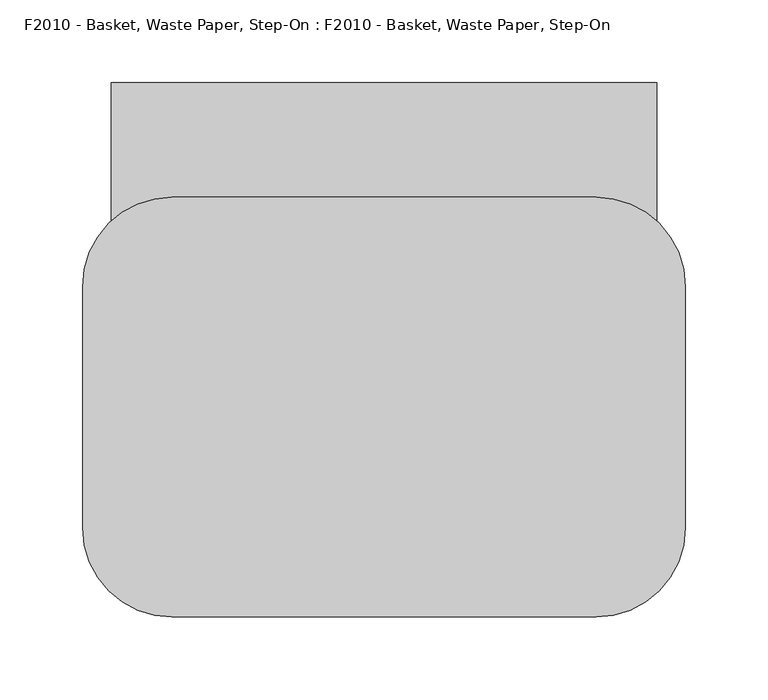
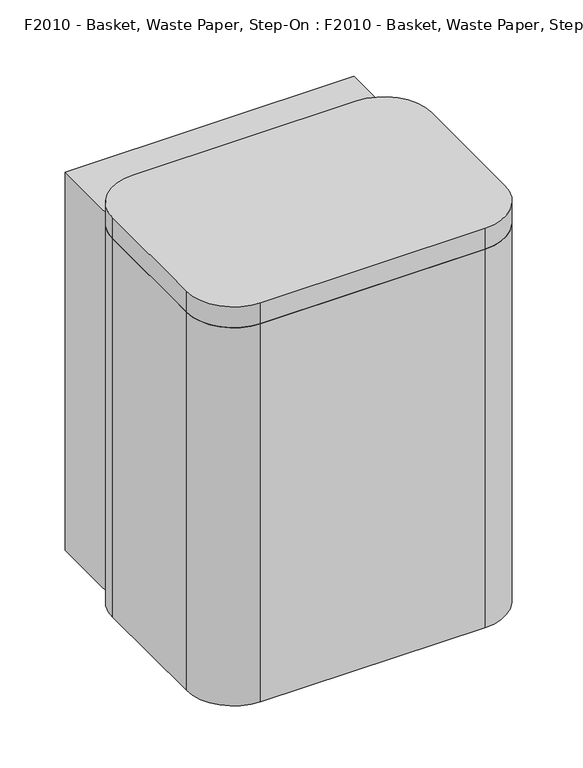
"""IFC4 building model written with IfcOpenShell, lengths in millimetres: proxy geometry, F2010 - Basket, Waste Paper, Step-On : F2010 - Basket, Waste Paper, Step-On."""

import ifcopenshell
import ifcopenshell.guid

model = None  # the IFC model being written
_history = None  # IfcOwnerHistory: only IFC2X3 demands one
_inside = {}  # id of a spatial element -> (the spatial element, [elements in it])
_under = {}  # id of a project, library or spatial element -> (it, [spatial elements below it])
_declared = {}  # id of a project -> (the project, [libraries it declares])
_typed = {}  # id of a type object -> (the type object, [elements of that type])
_made_of = {}  # id of a material, layer set ... -> (it, [elements and type objects made of it])


def new_model(schema):
    """Start an empty IFC model of exactly this schema.

    Asked for "IFC4X3", IfcOpenShell would pick the latest addendum, in which some entities
    have other attributes; the version numbers below select the first issue.
    IFC2X3 requires an IfcOwnerHistory on every rooted entity: one is made here for all.
    """
    global model, _history
    if schema == "IFC4X3":
        model = ifcopenshell.file(schema_version=(4, 3, 0, 0))
    else:
        model = ifcopenshell.file(schema=schema)
    _inside.clear()
    _under.clear()
    _declared.clear()
    _typed.clear()
    _made_of.clear()
    _history = None
    if model.schema == "IFC2X3":
        org = make("IfcOrganization", Name="unknown")
        user = make(
            "IfcPersonAndOrganization",
            ThePerson=make("IfcPerson", FamilyName="unknown"),
            TheOrganization=org,
        )
        app = make(
            "IfcApplication",
            ApplicationDeveloper=org,
            Version="unknown",
            ApplicationFullName="unknown",
            ApplicationIdentifier="unknown",
        )
        _history = make(
            "IfcOwnerHistory",
            OwningUser=user,
            OwningApplication=app,
            ChangeAction="ADDED",
            CreationDate=0,
        )
    return model


def make(cls, **values):
    """One entity of the class cls with the attributes given. An attribute that is None is left unset."""
    return model.create_entity(
        cls, **{name: value for name, value in values.items() if value is not None}
    )


def rooted(cls, **values):
    """An entity with a GlobalId (a new one), such as an element, a storey or a relation."""
    return make(cls, GlobalId=ifcopenshell.guid.new(), OwnerHistory=_history, **values)


def si_unit(unit_type, name, prefix=None):
    """IfcSIUnit, for example si_unit("LENGTHUNIT", "METRE", prefix="MILLI")."""
    return make("IfcSIUnit", UnitType=unit_type, Prefix=prefix, Name=name)


def assignment(units):
    """IfcUnitAssignment: the units of a project."""
    return None if units is None else make("IfcUnitAssignment", Units=units)


def point(xyz):
    """IfcCartesianPoint."""
    return None if xyz is None else make("IfcCartesianPoint", Coordinates=xyz)


def direction(xyz):
    """IfcDirection."""
    return None if xyz is None else make("IfcDirection", DirectionRatios=xyz)


def frame(location, z_axis=None, x_axis=None):
    """IfcAxis2Placement3D, a coordinate frame: its origin and axes. An axis left out is left unset."""
    return make(
        "IfcAxis2Placement3D",
        Location=point(location),
        Axis=direction(z_axis),
        RefDirection=direction(x_axis),
    )


def frame_2d(location, x_axis=None):
    """IfcAxis2Placement2D, a coordinate frame in the plane: its origin and x axis."""
    return make(
        "IfcAxis2Placement2D", Location=point(location), RefDirection=direction(x_axis)
    )


def origin():
    """The frame at (0, 0, 0) with its axes left unset."""
    return frame((0.0, 0.0, 0.0))


def origin_with_axes():
    """The frame at (0, 0, 0) with the z axis (0, 0, 1) and the x axis (1, 0, 0) written out."""
    return frame((0.0, 0.0, 0.0), z_axis=(0.0, 0.0, 1.0), x_axis=(1.0, 0.0, 0.0))


def place(relative_to, where):
    """IfcLocalPlacement: puts the frame where relative to a parent placement (None: the world)."""
    return make(
        "IfcLocalPlacement", PlacementRelTo=relative_to, RelativePlacement=where
    )


def context(
    kind, dimensions, precision=None, world=None, true_north=None, identifier=None
):
    """IfcGeometricRepresentationContext, for example the 3D "Model" context."""
    return make(
        "IfcGeometricRepresentationContext",
        ContextIdentifier=identifier,
        ContextType=kind,
        CoordinateSpaceDimension=dimensions,
        Precision=precision,
        WorldCoordinateSystem=world,
        TrueNorth=true_north,
    )


def project(units=None, contexts=None):
    """IfcProject with its units and contexts."""
    return rooted(
        "IfcProject",
        Name="project",
        RepresentationContexts=contexts,
        UnitsInContext=assignment(units),
    )


def spatial(cls, under=None, at=None, **own):
    """A site, building, storey or space (cls), placed at a placement, below another one or the project."""
    s = rooted(cls, ObjectPlacement=at, **own)
    if under is not None:
        _under.setdefault(under.id(), (under, []))[1].append(s)
    return s


def polyline(points):
    """IfcPolyline through the points."""
    return make("IfcPolyline", Points=[point(p) for p in points])


def circle_curve(where, radius):
    """IfcCircle in the frame where."""
    return make("IfcCircle", Position=where, Radius=radius)


def trimmed(basis, trim1, trim2, sense, master):
    """IfcTrimmedCurve: the piece of a basis curve between two trims."""
    return make(
        "IfcTrimmedCurve",
        BasisCurve=basis,
        Trim1=trim1,
        Trim2=trim2,
        SenseAgreement=sense,
        MasterRepresentation=master,
    )


def segment(curve, same_sense, transition):
    """IfcCompositeCurveSegment."""
    return make(
        "IfcCompositeCurveSegment",
        Transition=transition,
        SameSense=same_sense,
        ParentCurve=curve,
    )


def composite_curve(segments, self_intersect=None):
    """IfcCompositeCurve: segments joined end to end."""
    return make("IfcCompositeCurve", Segments=segments, SelfIntersect=self_intersect)


def outline(outer, holes=None, kind="AREA"):
    """IfcArbitraryClosedProfileDef: a profile drawn as a closed curve; with holes, ...WithVoids."""
    if holes is None:
        return make("IfcArbitraryClosedProfileDef", ProfileType=kind, OuterCurve=outer)
    return make(
        "IfcArbitraryProfileDefWithVoids",
        ProfileType=kind,
        OuterCurve=outer,
        InnerCurves=holes,
    )


def extrude(swept, where, along, depth):
    """IfcExtrudedAreaSolid: the profile swept, set in the frame where, extruded along a direction by depth."""
    return make(
        "IfcExtrudedAreaSolid",
        SweptArea=swept,
        Position=where,
        ExtrudedDirection=direction(along),
        Depth=depth,
    )


def shape(context_of_items, identifier, shape_type, items):
    """IfcShapeRepresentation: the items that make up one representation, for example the "Body"."""
    return make(
        "IfcShapeRepresentation",
        ContextOfItems=context_of_items,
        RepresentationIdentifier=identifier,
        RepresentationType=shape_type,
        Items=items,
    )


def source(mapping_origin, context_of_items, identifier, shape_type, items):
    """IfcRepresentationMap: a shape defined once, which mapped items show again and again."""
    return make(
        "IfcRepresentationMap",
        MappingOrigin=mapping_origin,
        MappedRepresentation=shape(context_of_items, identifier, shape_type, items),
    )


def transform(
    local_origin,
    x_axis=None,
    y_axis=None,
    z_axis=None,
    scale=None,
    scale2=None,
    scale3=None,
    uniform=True,
):
    """IfcCartesianTransformationOperator3D, or its non-uniform kind. x_axis, y_axis, z_axis: its Axis1, 2, 3."""
    if uniform:
        return make(
            "IfcCartesianTransformationOperator3D",
            Axis1=direction(x_axis),
            Axis2=direction(y_axis),
            LocalOrigin=point(local_origin),
            Scale=scale,
            Axis3=direction(z_axis),
        )
    return make(
        "IfcCartesianTransformationOperator3DnonUniform",
        Axis1=direction(x_axis),
        Axis2=direction(y_axis),
        LocalOrigin=point(local_origin),
        Scale=scale,
        Axis3=direction(z_axis),
        Scale2=scale2,
        Scale3=scale3,
    )


def mapped(mapping_source, mapping_target):
    """IfcMappedItem: shows the shape of a source again, moved by a transform."""
    return make(
        "IfcMappedItem", MappingSource=mapping_source, MappingTarget=mapping_target
    )


def made_of(thing, what):
    """Note that an element or type object is made of a material, layer set ...; save() writes the relation."""
    if what is not None:
        _made_of.setdefault(what.id(), (what, []))[1].append(thing)
    return thing


def element(
    cls,
    number,
    at=None,
    inside=None,
    cuts=None,
    type_object=None,
    material=None,
    context=None,
    identifier="Body",
    shape_type=None,
    held_by="IfcProductDefinitionShape",
    body=None,
    shapes=None,
    **own,
):
    """One element of the class cls, such as IfcWall. Its Tag is "e" and its number.

    at: its placement. inside: the storey or other place that contains it. cuts: it is an
    opening in that element (IfcRelVoidsElement). A single representation is given by context,
    identifier, shape_type and body (its items); several are given by shapes. held_by: the class
    of the entity that holds the representations. save() writes the other relations.
    """
    e = rooted(cls, Tag="e%d" % number, ObjectPlacement=at, **own)
    if body is not None:
        shapes = [shape(context, identifier, shape_type, body)]
    if shapes is not None:
        e.Representation = make(held_by, Representations=shapes)
    if inside is not None:
        _inside.setdefault(inside.id(), (inside, []))[1].append(e)
    if cuts is not None:
        rooted(
            "IfcRelVoidsElement", RelatingBuildingElement=cuts, RelatedOpeningElement=e
        )
    if type_object is not None:
        _typed.setdefault(type_object.id(), (type_object, []))[1].append(e)
    return made_of(e, material)


def aggregate(whole, parts):
    """IfcRelAggregates: a whole, such as a stair, and the parts it consists of."""
    return rooted("IfcRelAggregates", RelatingObject=whole, RelatedObjects=parts)


def save(model, path):
    """Write the relations noted so far, then the file.

    IfcRelAggregates (storeys below a building ...), IfcRelContainedInSpatialStructure (elements
    in a storey), IfcRelDefinesByType, IfcRelAssociatesMaterial and IfcRelDeclares: one each for
    every whole, place, type object, material and project.
    """
    for whole, parts in _under.values():
        aggregate(whole, parts)
    for where, things in _inside.values():
        rooted(
            "IfcRelContainedInSpatialStructure",
            RelatedElements=things,
            RelatingStructure=where,
        )
    for kind, things in _typed.values():
        rooted("IfcRelDefinesByType", RelatedObjects=things, RelatingType=kind)
    for what, things in _made_of.values():
        rooted("IfcRelAssociatesMaterial", RelatedObjects=things, RelatingMaterial=what)
    for by, libraries in _declared.values():
        rooted("IfcRelDeclares", RelatingContext=by, RelatedDefinitions=libraries)
    model.write(path)


def plane_surface(at):
    """IfcPlane: the flat surface through the origin of the frame at, square to its z axis."""
    return make("IfcPlane", Position=at)


def cylinder_surface(at, radius):
    """IfcCylindricalSurface: all points at the distance radius from the z axis of the frame at."""
    return make("IfcCylindricalSurface", Position=at, Radius=radius)


def revolved_surface(curve, axis_point, axis_direction):
    """IfcSurfaceOfRevolution: the curve turned about the line through axis_point along axis_direction."""
    return make(
        "IfcSurfaceOfRevolution",
        SweptCurve=make("IfcArbitraryOpenProfileDef", ProfileType="CURVE", Curve=curve),
        AxisPosition=make("IfcAxis1Placement", Location=point(axis_point), Axis=direction(axis_direction)),
    )


def advanced_brep(points, edges, surfaces, faces):
    """IfcAdvancedBrep: a solid bounded by faces that lie on surfaces and meet in shared edges.

    An edge is (start, end): straight between two places in points (the first is 0);
    or (start, end, curve); or (start, end, curve, False) where it runs against its curve.
    A face is (place in surfaces, loops), or (place, loops, False) where it looks against
    its surface's normal. A loop lists edges by number (the first is 1), with a minus sign
    where the edge is run from its end to its start. The first loop is the outer one.
    """
    corners = [point(p) for p in points]
    vertices = [make("IfcVertexPoint", VertexGeometry=c) for c in corners]
    made = []
    for start, end, *more in edges:
        made.append(
            make(
                "IfcEdgeCurve",
                EdgeStart=vertices[start],
                EdgeEnd=vertices[end],
                EdgeGeometry=more[0] if more else make("IfcPolyline", Points=[corners[start], corners[end]]),
                SameSense=more[1] if len(more) > 1 else True,
            )
        )
    hull = []
    for where, loops, *sense in faces:
        bounds = []
        for j, loop in enumerate(loops):
            ring = [make("IfcOrientedEdge", EdgeElement=made[abs(k) - 1], Orientation=k > 0) for k in loop]
            bounds.append(
                make(
                    "IfcFaceOuterBound" if j == 0 else "IfcFaceBound",
                    Bound=make("IfcEdgeLoop", EdgeList=ring),
                    Orientation=True,
                )
            )
        hull.append(make("IfcAdvancedFace", Bounds=bounds, FaceSurface=surfaces[where], SameSense=sense[0] if sense else True))
    return make("IfcAdvancedBrep", Outer=make("IfcClosedShell", CfsFaces=hull))


def f2010_basket_waste_paper_step_on_f2010_basket_waste_paper_7402589c(model_context):
    return source(origin(), model_context, "Body", "SolidModel", [
        advanced_brep(
        [(128.266525, -170.9615385, 457.2), (182.241525, -116.9865385, 457.2), (182.241525, 29.0634615, 457.2), (128.266525, 83.0384615, 457.2), (-128.266525, 83.0384615, 457.2), (-182.241525, 29.0634615, 457.2), (-182.241525, -116.9865385, 457.2), (-128.266525, -170.9615385, 457.2), (-114.3, -164.6115385, 457.2), (-165.1, -113.8115385, 457.2), (-165.1, 25.8884615, 457.2), (-114.3, 76.6884615, 457.2), (114.3, 76.6884615, 457.2), (165.1, 25.8884615, 457.2), (165.1, -113.8115385, 457.2), (114.3, -164.6115385, 457.2), (128.266525, -170.9615385, 0.0), (-128.266525, -170.9615385, 0.0), (-182.241525, -116.9865385, 0.0), (-182.241525, 29.0634615, 0.0), (-128.266525, 83.0384615, 0.0), (128.266525, 83.0384615, 0.0), (182.241525, 29.0634615, 0.0), (182.241525, -116.9865385, 0.0), (114.3, -164.6115385, 12.7), (165.1, -113.8115385, 12.7), (165.1, 25.8884615, 12.7), (114.3, 76.6884615, 12.7), (-114.3, 76.6884615, 12.7), (-165.1, 25.8884615, 12.7), (-165.1, -113.8115385, 12.7), (-114.3, -164.6115385, 12.7)],
        [
            (0, 1, circle_curve(frame((128.266525, -116.9865385, 457.2), z_axis=(0.0, 0.0, 1.0), x_axis=(1.0, 0.0, 0.0)), 53.975)),
            (1, 2),
            (2, 3, circle_curve(frame((128.266525, 29.0634615, 457.2), z_axis=(0.0, 0.0, 1.0), x_axis=(1.0, 0.0, 0.0)), 53.975)),
            (3, 4),
            (4, 5, circle_curve(frame((-128.266525, 29.0634615, 457.2), z_axis=(0.0, 0.0, 1.0), x_axis=(1.0, 0.0, 0.0)), 53.975)),
            (5, 6),
            (6, 7, circle_curve(frame((-128.266525, -116.9865385, 457.2), z_axis=(0.0, 0.0, 1.0), x_axis=(1.0, 0.0, 0.0)), 53.975)),
            (7, 0),
            (8, 9, circle_curve(frame((-114.3, -113.8115385, 457.2), z_axis=(0.0, 0.0, -1.0), x_axis=(1.0, 0.0, 0.0)), 50.8)),
            (9, 10),
            (10, 11, circle_curve(frame((-114.3, 25.8884615, 457.2), z_axis=(0.0, 0.0, -1.0), x_axis=(1.0, 0.0, 0.0)), 50.8)),
            (11, 12),
            (12, 13, circle_curve(frame((114.3, 25.8884615, 457.2), z_axis=(0.0, 0.0, -1.0), x_axis=(1.0, 0.0, 0.0)), 50.8)),
            (13, 14),
            (14, 15, circle_curve(frame((114.3, -113.8115385, 457.2), z_axis=(0.0, 0.0, -1.0), x_axis=(1.0, 0.0, 0.0)), 50.8)),
            (15, 8),
            (16, 17),
            (17, 18, circle_curve(frame((-128.266525, -116.9865385, 0.0), z_axis=(0.0, 0.0, -1.0), x_axis=(1.0, 0.0, 0.0)), 53.975)),
            (18, 19),
            (19, 20, circle_curve(frame((-128.266525, 29.0634615, 0.0), z_axis=(0.0, 0.0, -1.0), x_axis=(1.0, 0.0, 0.0)), 53.975)),
            (20, 21),
            (21, 22, circle_curve(frame((128.266525, 29.0634615, 0.0), z_axis=(0.0, 0.0, -1.0), x_axis=(1.0, 0.0, 0.0)), 53.975)),
            (22, 23),
            (23, 16, circle_curve(frame((128.266525, -116.9865385, 0.0), z_axis=(0.0, 0.0, -1.0), x_axis=(1.0, 0.0, 0.0)), 53.975)),
            (7, 17),
            (16, 0),
            (6, 18),
            (5, 19),
            (4, 20),
            (3, 21),
            (2, 22),
            (1, 23),
            (24, 25, circle_curve(frame((114.3, -113.8115385, 12.7), z_axis=(0.0, 0.0, 1.0), x_axis=(1.0, 0.0, 0.0)), 50.8)),
            (25, 26),
            (26, 27, circle_curve(frame((114.3, 25.8884615, 12.7), z_axis=(0.0, 0.0, 1.0), x_axis=(1.0, 0.0, 0.0)), 50.8)),
            (27, 28),
            (28, 29, circle_curve(frame((-114.3, 25.8884615, 12.7), z_axis=(0.0, 0.0, 1.0), x_axis=(1.0, 0.0, 0.0)), 50.8)),
            (29, 30),
            (30, 31, circle_curve(frame((-114.3, -113.8115385, 12.7), z_axis=(0.0, 0.0, 1.0), x_axis=(1.0, 0.0, 0.0)), 50.8)),
            (31, 24),
            (31, 8),
            (15, 24),
            (30, 9),
            (29, 10),
            (28, 11),
            (27, 12),
            (26, 13),
            (25, 14),
        ],
        [
            plane_surface(frame((-182.241525, -170.9615385, 457.2), z_axis=(0.0, 0.0, 1.0), x_axis=(-1.0, 0.0, 0.0))),
            plane_surface(frame((-182.241525, -170.9615385, 0.0), z_axis=(0.0, 0.0, -1.0), x_axis=(1.0, 0.0, 0.0))),
            plane_surface(frame((128.266525, -170.9615385, 457.2), z_axis=(0.0, -1.0, 0.0), x_axis=(0.0, 0.0, -1.0))),
            cylinder_surface(frame((-128.266525, -116.9865385, 0.0), z_axis=(0.0, 0.0, 1.0), x_axis=(1.0, 0.0, 0.0)), 53.975),
            plane_surface(frame((-182.241525, -116.9865385, 457.2), z_axis=(-1.0, 0.0, 0.0), x_axis=(0.0, 0.0, -1.0))),
            cylinder_surface(frame((-128.266525, 29.0634615, 0.0), z_axis=(0.0, 0.0, 1.0), x_axis=(1.0, 0.0, 0.0)), 53.975),
            plane_surface(frame((-128.266525, 83.0384615, 457.2), z_axis=(0.0, 1.0, 0.0), x_axis=(0.0, 0.0, -1.0))),
            cylinder_surface(frame((128.266525, 29.0634615, 0.0), z_axis=(0.0, 0.0, 1.0), x_axis=(1.0, 0.0, 0.0)), 53.975),
            plane_surface(frame((182.241525, 29.0634615, 457.2), z_axis=(1.0, 0.0, 0.0), x_axis=(0.0, 0.0, -1.0))),
            cylinder_surface(frame((128.266525, -116.9865385, 0.0), z_axis=(0.0, 0.0, 1.0), x_axis=(1.0, 0.0, 0.0)), 53.975),
            plane_surface(frame((-125.091525, -164.6115385, 12.7), z_axis=(0.0, 0.0, 1.0), x_axis=(1.0, 0.0, 0.0))),
            plane_surface(frame((114.3, -164.6115385, 457.2), z_axis=(0.0, 1.0, 0.0), x_axis=(0.0, 0.0, -1.0))),
            revolved_surface(polyline([(-63.5, -113.8115385, 457.2), (-63.5, -113.8115385, 12.7)]), (-114.3, -113.8115385, 12.7), (0.0, 0.0, 1.0)),
            plane_surface(frame((-165.1, -113.8115385, 457.2), z_axis=(1.0, 0.0, 0.0), x_axis=(0.0, 0.0, -1.0))),
            revolved_surface(polyline([(-63.5, 25.8884615, 457.2), (-63.5, 25.8884615, 12.7)]), (-114.3, 25.8884615, 12.7), (0.0, 0.0, 1.0)),
            plane_surface(frame((-114.3, 76.6884615, 457.2), z_axis=(0.0, -1.0, 0.0), x_axis=(0.0, 0.0, -1.0))),
            revolved_surface(polyline([(165.1, 25.8884615, 457.2), (165.1, 25.8884615, 12.7)]), (114.3, 25.8884615, 12.7), (0.0, 0.0, 1.0)),
            plane_surface(frame((165.1, 25.8884615, 457.2), z_axis=(-1.0, 0.0, 0.0), x_axis=(0.0, 0.0, -1.0))),
            revolved_surface(polyline([(165.1, -113.8115385, 457.2), (165.1, -113.8115385, 12.7)]), (114.3, -113.8115385, 12.7), (0.0, 0.0, 1.0)),
        ],
        [
            (0, [[1, 2, 3, 4, 5, 6, 7, 8], [9, 10, 11, 12, 13, 14, 15, 16]]),
            (1, [[17, 18, 19, 20, 21, 22, 23, 24]]),
            (2, [[25, -17, 26, -8]]),
            (3, [[27, -18, -25, -7]]),
            (4, [[28, -19, -27, -6]]),
            (5, [[29, -20, -28, -5]]),
            (6, [[30, -21, -29, -4]]),
            (7, [[31, -22, -30, -3]]),
            (8, [[32, -23, -31, -2]]),
            (9, [[-26, -24, -32, -1]]),
            (10, [[33, 34, 35, 36, 37, 38, 39, 40]]),
            (11, [[41, -16, 42, -40]]),
            (12, [[43, -9, -41, -39]]),
            (13, [[44, -10, -43, -38]]),
            (14, [[45, -11, -44, -37]]),
            (15, [[46, -12, -45, -36]]),
            (16, [[47, -13, -46, -35]]),
            (17, [[48, -14, -47, -34]]),
            (18, [[-42, -15, -48, -33]]),
        ],
    ),
        extrude(outline(polyline([(50.8, 83.0384615), (50.8, 6.8384615), (-50.8, 6.8384615), (-50.8, 83.0384615), (50.8, 83.0384615)])), origin_with_axes(), (0.0, 0.0, 1.0), 105.5317808),
        extrude(outline(polyline([(38.1, 57.6384615), (-38.1, 57.6384615), (-38.1, 133.8384615), (38.1, 133.8384615), (38.1, 57.6384615)])), origin_with_axes(), (0.0, 0.0, 1.0), 50.8),
        extrude(outline(composite_curve([segment(polyline([(128.266525, -170.9615385), (-128.266525, -170.9615385)]), True, "CONTINUOUS"), segment(trimmed(circle_curve(frame_2d((-128.266525, -116.9865385)), 53.975), [point((-128.266525, -170.9615385))], [point((-182.241525, -116.9865385))], False, "CARTESIAN"), True, "CONTINUOUS"), segment(polyline([(-182.241525, -116.9865385), (-182.241525, 29.0634615)]), True, "CONTINUOUS"), segment(trimmed(circle_curve(frame_2d((-128.266525, 29.0634615)), 53.975), [point((-182.241525, 29.0634615))], [point((-128.266525, 83.0384615))], False, "CARTESIAN"), True, "CONTINUOUS"), segment(polyline([(-128.266525, 83.0384615), (128.266525, 83.0384615)]), True, "CONTINUOUS"), segment(trimmed(circle_curve(frame_2d((128.266525, 29.0634615)), 53.975), [point((128.266525, 83.0384615))], [point((182.241525, 29.0634615))], False, "CARTESIAN"), True, "CONTINUOUS"), segment(polyline([(182.241525, 29.0634615), (182.241525, -116.9865385)]), True, "CONTINUOUS"), segment(trimmed(circle_curve(frame_2d((128.266525, -116.9865385)), 53.975), [point((182.241525, -116.9865385))], [point((128.266525, -170.9615385))], False, "CARTESIAN"), True, "CONTINUOUS")], self_intersect=False)), frame((0.0, 0.0, 457.2), z_axis=(0.0, 0.0, 1.0), x_axis=(1.0, 0.0, 0.0)), (0.0, 0.0, 1.0), 25.4),
        extrude(outline(polyline([(-165.1, -152.4), (-165.1, 0.0), (-165.1, 152.4), (165.1, 152.4), (165.1, -152.4), (-165.1, -152.4)])), origin_with_axes(), (0.0, 0.0, 1.0), 457.2),
    ])


if __name__ == "__main__":
    model = new_model("IFC4")
    model_context = context("Model", 3, world=origin())
    ifc_project = project(units=[si_unit("LENGTHUNIT", "METRE", prefix="MILLI")], contexts=[model_context])
    site = spatial("IfcSite", under=ifc_project)
    building = spatial("IfcBuilding", under=site)
    placement = place(None, origin())
    f2010_basket_waste_paper_step_on_f2010_basket_waste_paper_shape = f2010_basket_waste_paper_step_on_f2010_basket_waste_paper_7402589c(model_context)
    element("IfcBuildingElementProxy", 1, Name="F2010 - Basket, Waste Paper, Step-On : F2010 - Basket, Waste Paper, Step-On", ObjectType="F2010 - Basket, Waste Paper, Step-On : F2010 - Basket, Waste Paper, Step-On", at=placement, inside=building, context=model_context, shape_type="MappedRepresentation", body=[
        mapped(f2010_basket_waste_paper_step_on_f2010_basket_waste_paper_shape, transform((0.0, 0.0, 0.0), x_axis=(1.0, 0.0, 0.0), y_axis=(0.0, 1.0, 0.0), z_axis=(0.0, 0.0, 1.0))),
    ])
    save(model, "model.ifc")

# Revit data of these elements
# Project information
#   Room Abbreviation = "NYIR1/NYAR1"
#   Room Description 2-1 = "Bedroom, Nursery, Airborne Infection Isolation (NYIR1)"
#   Room Description 2-2 = "Anteroom, Nursery, Airborne Infection Isolation (NYAR1)"
#   Sheets - Total = "6"
#   Project Issue Date = "Issue Date"
#   Project Status = "Project Status"
#   Client Name = "Owner"
#   Project Address = "Enter address here"
#   Project Name = "Project Name"
#   Project Number = "Project Number"
#   Publication Date = "30-Jan-15"
# Type "F2010 - Basket, Waste Paper, Step-On : F2010 - Basket, Waste Paper, Step-On"
#   Watts2 = "0"
#   Watts1 = "0"
#   Unit_Issue = "EA"
#   UTIL_6_Misc = "-"
#   UTIL_5_NonMedGas = "-"
#   UTIL_4_MiscGas = "-"
#   UTIL_3_MedGas = "-"
#   UTIL_2_Elec = "-"
#   UTIL_1_WaterDrain = "-"
#   Nomenclature = "Basket, Wastepaper, Step-On"
#   NSN = "7240007883953"
#   Location [instance default] = ""
#   JSN = "F2010"
#   Fund_Source_VA = "-"
#   Fund_Source_Navy = "-"
#   Fund_Source_Army = "-"
#   Fund_Source_AF = "-"
#   ELEC_Volts2 = "0"
#   ELEC_Volts1 = "0"
#   ELEC_Phase2 = "0"
#   ELEC_Phase1 = "0"
#   ELEC_HertzSwitch = "0"
#   ELEC_HertzDependent = "0"
#   ELEC_Hertz = "0"
#   ELEC_Amps2 = "0"
#   ELEC_Amps1 = "0"
#   DetailDescription = "\"Step-on\" wastepaper basket with inner liner and foot petal activated flip top."
#   CAT_VA = "C"
#   CAT_Navy = "C"
#   CAT_IHS = "-"
#   CAT_Army = "C"
#   CAT_AF = "C"
#   BTUperhour = "0"
#   Weight_IP = 12
#   DIM_Width_IP = 1' - 1"
#   DIM_Height_IP = 1' - 6"
#   DIM_Depth_IP = 1' - 0"
# Element 1 (IfcBuildingElementProxy, "F2010 - Basket, Waste Paper, Step-On : F2010 - Basket, Waste Paper, Step-On")
#   Location = "NYAR1"
#   Materials on its faces: "Metal - Chrome", "EquipSpace"
# Materials
#   "Metal - Chrome": class "Metal", colour RGB 17 17 17, transparency 0
#   "EquipSpace": class "Unassigned", colour RGB 221 217 195, transparency 0.5
